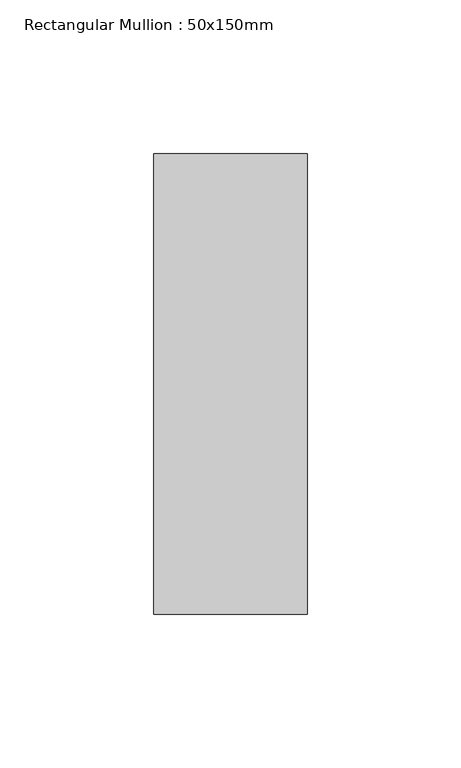
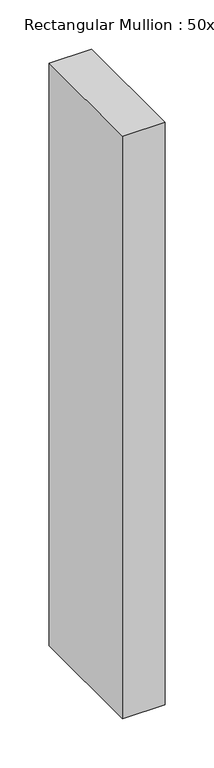
"""IFC4 building model written with IfcOpenShell, lengths in millimetres: member geometry, Rectangular Mullion : 50x150mm."""

from ifc_helpers import new_model, si_unit, frame, origin, place, context, project, spatial, polyline, outline, extrude, source, transform, mapped, element, save


def rectangular_mullion_50x150mm_74263cd1(model_context):
    return source(origin(), model_context, "Body", "SweptSolid", [
        extrude(outline(polyline([(0.0, 75.0), (0.0, -75.0), (-50.0, -75.0), (-50.0, 75.0), (0.0, 75.0)])), frame((0.0, 0.0, -725.0), z_axis=(0.0, 0.0, 1.0), x_axis=(1.0, 0.0, 0.0)), (0.0, 0.0, 1.0), 725.0),
    ])


if __name__ == "__main__":
    model = new_model("IFC4")
    model_context = context("Model", 3, world=origin())
    ifc_project = project(units=[si_unit("LENGTHUNIT", "METRE", prefix="MILLI")], contexts=[model_context])
    site = spatial("IfcSite", under=ifc_project)
    building = spatial("IfcBuilding", under=site)
    placement = place(None, origin())
    rectangular_mullion_50x150mm_shape = rectangular_mullion_50x150mm_74263cd1(model_context)
    element("IfcMember", 1, ObjectType="Rectangular Mullion : 50x150mm", at=placement, inside=building, context=model_context, shape_type="MappedRepresentation", body=[
        mapped(rectangular_mullion_50x150mm_shape, transform((0.0, 0.0, 0.0), x_axis=(1.0, 0.0, 0.0), y_axis=(0.0, 1.0, 0.0), z_axis=(0.0, 0.0, 1.0))),
    ])
    save(model, "model.ifc")

# Revit data of these elements
# Type "Rectangular Mullion : 50x150mm"
#   Keynote = "H11"
#   built-in parameter 1007304 = 0.492126 (stored number, unit not read)
#   built-in parameter 1007301 = 0.082021 (stored number, unit not read)
#   built-in parameter 1007300 = 0.082021 (stored number, unit not read)
# Element 1 (IfcMember, "Rectangular Mullion : 50x150mm")
#   Materials on its faces: "Aluminium"
# Materials
#   "Aluminium": class "Metal", colour RGB 247 247 247, transparency 0, Description = "Aluminium 6061", Cost = 0
